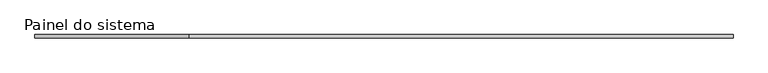
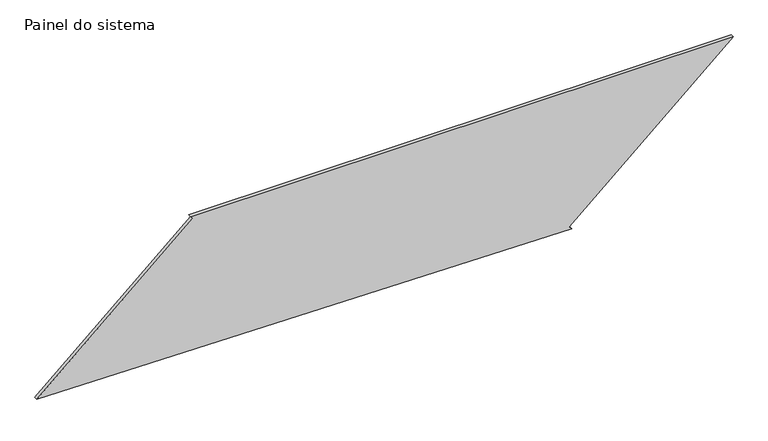
"""IFC4 building model written with IfcOpenShell, lengths in millimetres: plate geometry, Painel do sistema : Envidraçado."""

import ifcopenshell
import ifcopenshell.guid

model = None  # the IFC model being written
_history = None  # IfcOwnerHistory: only IFC2X3 demands one
_inside = {}  # id of a spatial element -> (the spatial element, [elements in it])
_under = {}  # id of a project, library or spatial element -> (it, [spatial elements below it])
_declared = {}  # id of a project -> (the project, [libraries it declares])
_typed = {}  # id of a type object -> (the type object, [elements of that type])
_made_of = {}  # id of a material, layer set ... -> (it, [elements and type objects made of it])


def new_model(schema):
    """Start an empty IFC model of exactly this schema.

    Asked for "IFC4X3", IfcOpenShell would pick the latest addendum, in which some entities
    have other attributes; the version numbers below select the first issue.
    IFC2X3 requires an IfcOwnerHistory on every rooted entity: one is made here for all.
    """
    global model, _history
    if schema == "IFC4X3":
        model = ifcopenshell.file(schema_version=(4, 3, 0, 0))
    else:
        model = ifcopenshell.file(schema=schema)
    _inside.clear()
    _under.clear()
    _declared.clear()
    _typed.clear()
    _made_of.clear()
    _history = None
    if model.schema == "IFC2X3":
        org = make("IfcOrganization", Name="unknown")
        user = make(
            "IfcPersonAndOrganization",
            ThePerson=make("IfcPerson", FamilyName="unknown"),
            TheOrganization=org,
        )
        app = make(
            "IfcApplication",
            ApplicationDeveloper=org,
            Version="unknown",
            ApplicationFullName="unknown",
            ApplicationIdentifier="unknown",
        )
        _history = make(
            "IfcOwnerHistory",
            OwningUser=user,
            OwningApplication=app,
            ChangeAction="ADDED",
            CreationDate=0,
        )
    return model


def make(cls, **values):
    """One entity of the class cls with the attributes given. An attribute that is None is left unset."""
    return model.create_entity(
        cls, **{name: value for name, value in values.items() if value is not None}
    )


def rooted(cls, **values):
    """An entity with a GlobalId (a new one), such as an element, a storey or a relation."""
    return make(cls, GlobalId=ifcopenshell.guid.new(), OwnerHistory=_history, **values)


def si_unit(unit_type, name, prefix=None):
    """IfcSIUnit, for example si_unit("LENGTHUNIT", "METRE", prefix="MILLI")."""
    return make("IfcSIUnit", UnitType=unit_type, Prefix=prefix, Name=name)


def assignment(units):
    """IfcUnitAssignment: the units of a project."""
    return None if units is None else make("IfcUnitAssignment", Units=units)


def point(xyz):
    """IfcCartesianPoint."""
    return None if xyz is None else make("IfcCartesianPoint", Coordinates=xyz)


def direction(xyz):
    """IfcDirection."""
    return None if xyz is None else make("IfcDirection", DirectionRatios=xyz)


def frame(location, z_axis=None, x_axis=None):
    """IfcAxis2Placement3D, a coordinate frame: its origin and axes. An axis left out is left unset."""
    return make(
        "IfcAxis2Placement3D",
        Location=point(location),
        Axis=direction(z_axis),
        RefDirection=direction(x_axis),
    )


def origin():
    """The frame at (0, 0, 0) with its axes left unset."""
    return frame((0.0, 0.0, 0.0))


def place(relative_to, where):
    """IfcLocalPlacement: puts the frame where relative to a parent placement (None: the world)."""
    return make(
        "IfcLocalPlacement", PlacementRelTo=relative_to, RelativePlacement=where
    )


def context(
    kind, dimensions, precision=None, world=None, true_north=None, identifier=None
):
    """IfcGeometricRepresentationContext, for example the 3D "Model" context."""
    return make(
        "IfcGeometricRepresentationContext",
        ContextIdentifier=identifier,
        ContextType=kind,
        CoordinateSpaceDimension=dimensions,
        Precision=precision,
        WorldCoordinateSystem=world,
        TrueNorth=true_north,
    )


def project(units=None, contexts=None):
    """IfcProject with its units and contexts."""
    return rooted(
        "IfcProject",
        Name="project",
        RepresentationContexts=contexts,
        UnitsInContext=assignment(units),
    )


def spatial(cls, under=None, at=None, **own):
    """A site, building, storey or space (cls), placed at a placement, below another one or the project."""
    s = rooted(cls, ObjectPlacement=at, **own)
    if under is not None:
        _under.setdefault(under.id(), (under, []))[1].append(s)
    return s


def polyline(points):
    """IfcPolyline through the points."""
    return make("IfcPolyline", Points=[point(p) for p in points])


def outline(outer, holes=None, kind="AREA"):
    """IfcArbitraryClosedProfileDef: a profile drawn as a closed curve; with holes, ...WithVoids."""
    if holes is None:
        return make("IfcArbitraryClosedProfileDef", ProfileType=kind, OuterCurve=outer)
    return make(
        "IfcArbitraryProfileDefWithVoids",
        ProfileType=kind,
        OuterCurve=outer,
        InnerCurves=holes,
    )


def extrude(swept, where, along, depth):
    """IfcExtrudedAreaSolid: the profile swept, set in the frame where, extruded along a direction by depth."""
    return make(
        "IfcExtrudedAreaSolid",
        SweptArea=swept,
        Position=where,
        ExtrudedDirection=direction(along),
        Depth=depth,
    )


def shape(context_of_items, identifier, shape_type, items):
    """IfcShapeRepresentation: the items that make up one representation, for example the "Body"."""
    return make(
        "IfcShapeRepresentation",
        ContextOfItems=context_of_items,
        RepresentationIdentifier=identifier,
        RepresentationType=shape_type,
        Items=items,
    )


def source(mapping_origin, context_of_items, identifier, shape_type, items):
    """IfcRepresentationMap: a shape defined once, which mapped items show again and again."""
    return make(
        "IfcRepresentationMap",
        MappingOrigin=mapping_origin,
        MappedRepresentation=shape(context_of_items, identifier, shape_type, items),
    )


def transform(
    local_origin,
    x_axis=None,
    y_axis=None,
    z_axis=None,
    scale=None,
    scale2=None,
    scale3=None,
    uniform=True,
):
    """IfcCartesianTransformationOperator3D, or its non-uniform kind. x_axis, y_axis, z_axis: its Axis1, 2, 3."""
    if uniform:
        return make(
            "IfcCartesianTransformationOperator3D",
            Axis1=direction(x_axis),
            Axis2=direction(y_axis),
            LocalOrigin=point(local_origin),
            Scale=scale,
            Axis3=direction(z_axis),
        )
    return make(
        "IfcCartesianTransformationOperator3DnonUniform",
        Axis1=direction(x_axis),
        Axis2=direction(y_axis),
        LocalOrigin=point(local_origin),
        Scale=scale,
        Axis3=direction(z_axis),
        Scale2=scale2,
        Scale3=scale3,
    )


def mapped(mapping_source, mapping_target):
    """IfcMappedItem: shows the shape of a source again, moved by a transform."""
    return make(
        "IfcMappedItem", MappingSource=mapping_source, MappingTarget=mapping_target
    )


def made_of(thing, what):
    """Note that an element or type object is made of a material, layer set ...; save() writes the relation."""
    if what is not None:
        _made_of.setdefault(what.id(), (what, []))[1].append(thing)
    return thing


def element(
    cls,
    number,
    at=None,
    inside=None,
    cuts=None,
    type_object=None,
    material=None,
    context=None,
    identifier="Body",
    shape_type=None,
    held_by="IfcProductDefinitionShape",
    body=None,
    shapes=None,
    **own,
):
    """One element of the class cls, such as IfcWall. Its Tag is "e" and its number.

    at: its placement. inside: the storey or other place that contains it. cuts: it is an
    opening in that element (IfcRelVoidsElement). A single representation is given by context,
    identifier, shape_type and body (its items); several are given by shapes. held_by: the class
    of the entity that holds the representations. save() writes the other relations.
    """
    e = rooted(cls, Tag="e%d" % number, ObjectPlacement=at, **own)
    if body is not None:
        shapes = [shape(context, identifier, shape_type, body)]
    if shapes is not None:
        e.Representation = make(held_by, Representations=shapes)
    if inside is not None:
        _inside.setdefault(inside.id(), (inside, []))[1].append(e)
    if cuts is not None:
        rooted(
            "IfcRelVoidsElement", RelatingBuildingElement=cuts, RelatedOpeningElement=e
        )
    if type_object is not None:
        _typed.setdefault(type_object.id(), (type_object, []))[1].append(e)
    return made_of(e, material)


def aggregate(whole, parts):
    """IfcRelAggregates: a whole, such as a stair, and the parts it consists of."""
    return rooted("IfcRelAggregates", RelatingObject=whole, RelatedObjects=parts)


def save(model, path):
    """Write the relations noted so far, then the file.

    IfcRelAggregates (storeys below a building ...), IfcRelContainedInSpatialStructure (elements
    in a storey), IfcRelDefinesByType, IfcRelAssociatesMaterial and IfcRelDeclares: one each for
    every whole, place, type object, material and project.
    """
    for whole, parts in _under.values():
        aggregate(whole, parts)
    for where, things in _inside.values():
        rooted(
            "IfcRelContainedInSpatialStructure",
            RelatedElements=things,
            RelatingStructure=where,
        )
    for kind, things in _typed.values():
        rooted("IfcRelDefinesByType", RelatedObjects=things, RelatingType=kind)
    for what, things in _made_of.values():
        rooted("IfcRelAssociatesMaterial", RelatedObjects=things, RelatingMaterial=what)
    for by, libraries in _declared.values():
        rooted("IfcRelDeclares", RelatingContext=by, RelatedDefinitions=libraries)
    model.write(path)


def painel_do_sistema_aae2b681(model_context):
    return source(origin(), model_context, "Body", "SweptSolid", [
        extrude(outline(polyline([(0.0, 1330.2468179), (18.8079041, 1313.7767619), (1041.3238686, 2481.4341349), (1041.3238686, -1385.6276252), (1022.5159645, -1369.1575693), (48.4968973, -2481.4341349), (0.0, 1330.2468179)])), frame((0.0, 24.5, 0.0), z_axis=(0.0, 1.0, 0.0), x_axis=(0.0, 0.0, 1.0)), (0.0, 0.0, 1.0), 25.0),
    ])


if __name__ == "__main__":
    model = new_model("IFC4")
    model_context = context("Model", 3, world=origin())
    ifc_project = project(units=[si_unit("LENGTHUNIT", "METRE", prefix="MILLI")], contexts=[model_context])
    site = spatial("IfcSite", under=ifc_project)
    building = spatial("IfcBuilding", under=site)
    placement = place(None, origin())
    painel_do_sistema_shape = painel_do_sistema_aae2b681(model_context)
    element("IfcPlate", 1, ObjectType="Painel do sistema : Envidraçado", at=placement, inside=building, context=model_context, shape_type="MappedRepresentation", body=[
        mapped(painel_do_sistema_shape, transform((0.0, 0.0, 0.0), x_axis=(1.0, 0.0, 0.0), y_axis=(0.0, 1.0, 0.0), z_axis=(0.0, 0.0, 1.0))),
    ])
    save(model, "model.ifc")

# Revit data of these elements
# Type "Painel do sistema : Envidraçado"
#   Construction Type Id = "GSP4R"
#   Analytic Construction = "Vidraça única Pilkington 1/8 pol"
#   Visual Light Transmittance = 0.9
#   Solar Heat Gain Coefficient = 0.86
#   Heat Transfer Coefficient (U) = 6.7069 W/(m²·K)
# Element 1 (IfcPlate, "Painel do sistema : Envidraçado")
#   Materials on its faces: "Vidro"
# Materials
#   "Vidro": class "Vidro", colour RGB 0 128 192, transparency 0.9, Description = "Vidro de sílica", Cost = 0
